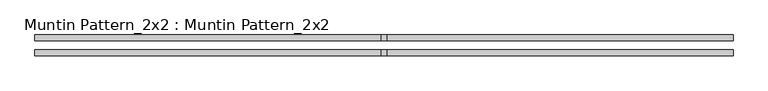
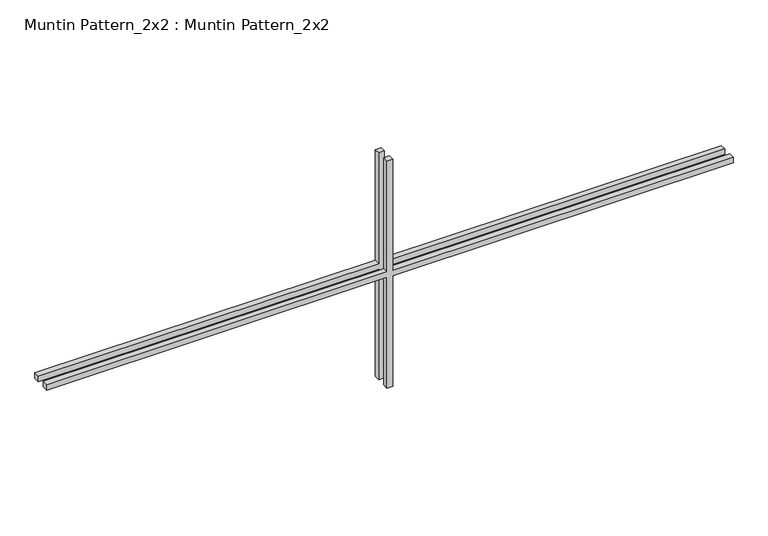
"""IFC4 building model written with IfcOpenShell, lengths in millimetres: proxy geometry, Muntin Pattern_2x2 : Muntin Pattern_2x2."""

from ifc_helpers import new_model, si_unit, frame, origin, place, context, project, spatial, polyline, outline, extrude, source, transform, mapped, element, save


def muntin_pattern_2x2_muntin_pattern_2x2_54380e04(model_context):
    return source(origin(), model_context, "Body", "SweptSolid", [
        extrude(outline(polyline([(268.2875, -6.35), (268.2875, -749.3), (255.5875, -749.3), (255.5875, -6.35), (0.0, -6.35), (0.0, 6.35), (255.5875, 6.35), (255.5875, 749.3), (268.2875, 749.3), (268.2875, 6.35), (523.875, 6.35), (523.875, -6.35), (268.2875, -6.35)])), frame((0.0, 9.525, 0.0), z_axis=(0.0, 1.0, 0.0), x_axis=(0.0, 0.0, 1.0)), (0.0, 0.0, 1.0), 12.7),
        extrude(outline(polyline([(268.2875, -6.35), (268.2875, -749.3), (255.5875, -749.3), (255.5875, -6.35), (0.0, -6.35), (0.0, 6.35), (255.5875, 6.35), (255.5875, 749.3), (268.2875, 749.3), (268.2875, 6.35), (523.875, 6.35), (523.875, -6.35), (268.2875, -6.35)])), frame((0.0, -22.225, 0.0), z_axis=(0.0, 1.0, 0.0), x_axis=(0.0, 0.0, 1.0)), (0.0, 0.0, 1.0), 12.7),
    ])


if __name__ == "__main__":
    model = new_model("IFC4")
    model_context = context("Model", 3, world=origin())
    ifc_project = project(units=[si_unit("LENGTHUNIT", "METRE", prefix="MILLI")], contexts=[model_context])
    site = spatial("IfcSite", under=ifc_project)
    building = spatial("IfcBuilding", under=site)
    placement = place(None, origin())
    muntin_pattern_2x2_muntin_pattern_2x2_shape = muntin_pattern_2x2_muntin_pattern_2x2_54380e04(model_context)
    element("IfcBuildingElementProxy", 1, Name="Muntin Pattern_2x2 : Muntin Pattern_2x2", ObjectType="Muntin Pattern_2x2 : Muntin Pattern_2x2", at=placement, inside=building, context=model_context, shape_type="MappedRepresentation", body=[
        mapped(muntin_pattern_2x2_muntin_pattern_2x2_shape, transform((0.0, 0.0, 0.0), x_axis=(1.0, 0.0, 0.0), y_axis=(0.0, 1.0, 0.0), z_axis=(0.0, 0.0, 1.0))),
    ])
    save(model, "model.ifc")

# Revit data of these elements
# Type "Muntin Pattern_2x2 : Muntin Pattern_2x2"
#   Width [instance default] = 4' - 0"
#   Thickness = 0' - 0 1/2"
#   Height [instance default] = 4' - 0"
#   Distance = 0' - 0 3/4"
#   Interior Material [instance default] = none
#   Exterior Material [instance default] = none
# Element 1 (IfcBuildingElementProxy, "Muntin Pattern_2x2 : Muntin Pattern_2x2")
#   Width = 4' - 11"
#   Height = 1' - 8 5/8"
#   Interior Material = Wood - Stained
#   Exterior Material = Clad - White
#   Materials on its faces: "Clad - White", "Wood - Stained"
# Materials
#   "Clad - White": class "Wood", colour RGB 242 242 238, transparency 0, Cost = 0
#   "Wood - Stained": class "Wood", colour RGB 224 178 126, transparency 0, Cost = 0
